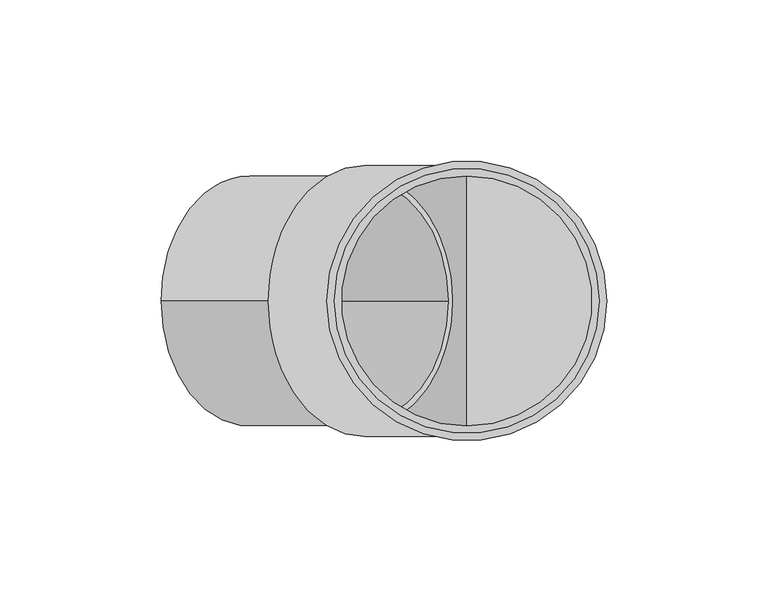
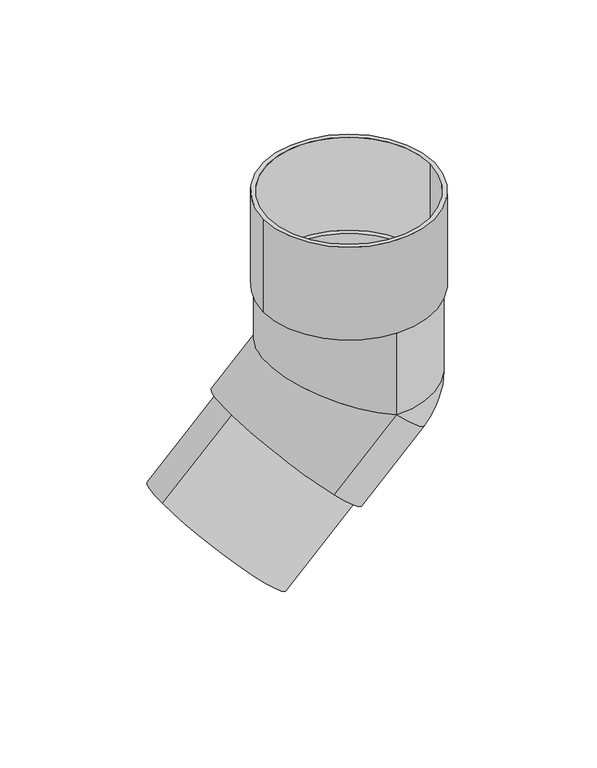
"""IFC4 building model written with IfcOpenShell, lengths in millimetres: proxy geometry, ⇲ Колено трубы 135 : ⇲ Колено трубы 135."""

import ifcopenshell
import ifcopenshell.guid

model = None  # the IFC model being written
_history = None  # IfcOwnerHistory: only IFC2X3 demands one
_inside = {}  # id of a spatial element -> (the spatial element, [elements in it])
_under = {}  # id of a project, library or spatial element -> (it, [spatial elements below it])
_declared = {}  # id of a project -> (the project, [libraries it declares])
_typed = {}  # id of a type object -> (the type object, [elements of that type])
_made_of = {}  # id of a material, layer set ... -> (it, [elements and type objects made of it])


def new_model(schema):
    """Start an empty IFC model of exactly this schema.

    Asked for "IFC4X3", IfcOpenShell would pick the latest addendum, in which some entities
    have other attributes; the version numbers below select the first issue.
    IFC2X3 requires an IfcOwnerHistory on every rooted entity: one is made here for all.
    """
    global model, _history
    if schema == "IFC4X3":
        model = ifcopenshell.file(schema_version=(4, 3, 0, 0))
    else:
        model = ifcopenshell.file(schema=schema)
    _inside.clear()
    _under.clear()
    _declared.clear()
    _typed.clear()
    _made_of.clear()
    _history = None
    if model.schema == "IFC2X3":
        org = make("IfcOrganization", Name="unknown")
        user = make(
            "IfcPersonAndOrganization",
            ThePerson=make("IfcPerson", FamilyName="unknown"),
            TheOrganization=org,
        )
        app = make(
            "IfcApplication",
            ApplicationDeveloper=org,
            Version="unknown",
            ApplicationFullName="unknown",
            ApplicationIdentifier="unknown",
        )
        _history = make(
            "IfcOwnerHistory",
            OwningUser=user,
            OwningApplication=app,
            ChangeAction="ADDED",
            CreationDate=0,
        )
    return model


def make(cls, **values):
    """One entity of the class cls with the attributes given. An attribute that is None is left unset."""
    return model.create_entity(
        cls, **{name: value for name, value in values.items() if value is not None}
    )


def rooted(cls, **values):
    """An entity with a GlobalId (a new one), such as an element, a storey or a relation."""
    return make(cls, GlobalId=ifcopenshell.guid.new(), OwnerHistory=_history, **values)


def si_unit(unit_type, name, prefix=None):
    """IfcSIUnit, for example si_unit("LENGTHUNIT", "METRE", prefix="MILLI")."""
    return make("IfcSIUnit", UnitType=unit_type, Prefix=prefix, Name=name)


def assignment(units):
    """IfcUnitAssignment: the units of a project."""
    return None if units is None else make("IfcUnitAssignment", Units=units)


def point(xyz):
    """IfcCartesianPoint."""
    return None if xyz is None else make("IfcCartesianPoint", Coordinates=xyz)


def direction(xyz):
    """IfcDirection."""
    return None if xyz is None else make("IfcDirection", DirectionRatios=xyz)


def frame(location, z_axis=None, x_axis=None):
    """IfcAxis2Placement3D, a coordinate frame: its origin and axes. An axis left out is left unset."""
    return make(
        "IfcAxis2Placement3D",
        Location=point(location),
        Axis=direction(z_axis),
        RefDirection=direction(x_axis),
    )


def origin():
    """The frame at (0, 0, 0) with its axes left unset."""
    return frame((0.0, 0.0, 0.0))


def origin_with_axes():
    """The frame at (0, 0, 0) with the z axis (0, 0, 1) and the x axis (1, 0, 0) written out."""
    return frame((0.0, 0.0, 0.0), z_axis=(0.0, 0.0, 1.0), x_axis=(1.0, 0.0, 0.0))


def place(relative_to, where):
    """IfcLocalPlacement: puts the frame where relative to a parent placement (None: the world)."""
    return make(
        "IfcLocalPlacement", PlacementRelTo=relative_to, RelativePlacement=where
    )


def context(
    kind, dimensions, precision=None, world=None, true_north=None, identifier=None
):
    """IfcGeometricRepresentationContext, for example the 3D "Model" context."""
    return make(
        "IfcGeometricRepresentationContext",
        ContextIdentifier=identifier,
        ContextType=kind,
        CoordinateSpaceDimension=dimensions,
        Precision=precision,
        WorldCoordinateSystem=world,
        TrueNorth=true_north,
    )


def project(units=None, contexts=None):
    """IfcProject with its units and contexts."""
    return rooted(
        "IfcProject",
        Name="project",
        RepresentationContexts=contexts,
        UnitsInContext=assignment(units),
    )


def spatial(cls, under=None, at=None, **own):
    """A site, building, storey or space (cls), placed at a placement, below another one or the project."""
    s = rooted(cls, ObjectPlacement=at, **own)
    if under is not None:
        _under.setdefault(under.id(), (under, []))[1].append(s)
    return s


def polyline(points):
    """IfcPolyline through the points."""
    return make("IfcPolyline", Points=[point(p) for p in points])


def circle_curve(where, radius):
    """IfcCircle in the frame where."""
    return make("IfcCircle", Position=where, Radius=radius)


def ellipse_curve(where, semi_axis1, semi_axis2):
    """IfcEllipse in the frame where."""
    return make(
        "IfcEllipse", Position=where, SemiAxis1=semi_axis1, SemiAxis2=semi_axis2
    )


def trimmed(basis, trim1, trim2, sense, master):
    """IfcTrimmedCurve: the piece of a basis curve between two trims."""
    return make(
        "IfcTrimmedCurve",
        BasisCurve=basis,
        Trim1=trim1,
        Trim2=trim2,
        SenseAgreement=sense,
        MasterRepresentation=master,
    )


def shape(context_of_items, identifier, shape_type, items):
    """IfcShapeRepresentation: the items that make up one representation, for example the "Body"."""
    return make(
        "IfcShapeRepresentation",
        ContextOfItems=context_of_items,
        RepresentationIdentifier=identifier,
        RepresentationType=shape_type,
        Items=items,
    )


def source(mapping_origin, context_of_items, identifier, shape_type, items):
    """IfcRepresentationMap: a shape defined once, which mapped items show again and again."""
    return make(
        "IfcRepresentationMap",
        MappingOrigin=mapping_origin,
        MappedRepresentation=shape(context_of_items, identifier, shape_type, items),
    )


def transform(
    local_origin,
    x_axis=None,
    y_axis=None,
    z_axis=None,
    scale=None,
    scale2=None,
    scale3=None,
    uniform=True,
):
    """IfcCartesianTransformationOperator3D, or its non-uniform kind. x_axis, y_axis, z_axis: its Axis1, 2, 3."""
    if uniform:
        return make(
            "IfcCartesianTransformationOperator3D",
            Axis1=direction(x_axis),
            Axis2=direction(y_axis),
            LocalOrigin=point(local_origin),
            Scale=scale,
            Axis3=direction(z_axis),
        )
    return make(
        "IfcCartesianTransformationOperator3DnonUniform",
        Axis1=direction(x_axis),
        Axis2=direction(y_axis),
        LocalOrigin=point(local_origin),
        Scale=scale,
        Axis3=direction(z_axis),
        Scale2=scale2,
        Scale3=scale3,
    )


def mapped(mapping_source, mapping_target):
    """IfcMappedItem: shows the shape of a source again, moved by a transform."""
    return make(
        "IfcMappedItem", MappingSource=mapping_source, MappingTarget=mapping_target
    )


def made_of(thing, what):
    """Note that an element or type object is made of a material, layer set ...; save() writes the relation."""
    if what is not None:
        _made_of.setdefault(what.id(), (what, []))[1].append(thing)
    return thing


def element(
    cls,
    number,
    at=None,
    inside=None,
    cuts=None,
    type_object=None,
    material=None,
    context=None,
    identifier="Body",
    shape_type=None,
    held_by="IfcProductDefinitionShape",
    body=None,
    shapes=None,
    **own,
):
    """One element of the class cls, such as IfcWall. Its Tag is "e" and its number.

    at: its placement. inside: the storey or other place that contains it. cuts: it is an
    opening in that element (IfcRelVoidsElement). A single representation is given by context,
    identifier, shape_type and body (its items); several are given by shapes. held_by: the class
    of the entity that holds the representations. save() writes the other relations.
    """
    e = rooted(cls, Tag="e%d" % number, ObjectPlacement=at, **own)
    if body is not None:
        shapes = [shape(context, identifier, shape_type, body)]
    if shapes is not None:
        e.Representation = make(held_by, Representations=shapes)
    if inside is not None:
        _inside.setdefault(inside.id(), (inside, []))[1].append(e)
    if cuts is not None:
        rooted(
            "IfcRelVoidsElement", RelatingBuildingElement=cuts, RelatedOpeningElement=e
        )
    if type_object is not None:
        _typed.setdefault(type_object.id(), (type_object, []))[1].append(e)
    return made_of(e, material)


def aggregate(whole, parts):
    """IfcRelAggregates: a whole, such as a stair, and the parts it consists of."""
    return rooted("IfcRelAggregates", RelatingObject=whole, RelatedObjects=parts)


def save(model, path):
    """Write the relations noted so far, then the file.

    IfcRelAggregates (storeys below a building ...), IfcRelContainedInSpatialStructure (elements
    in a storey), IfcRelDefinesByType, IfcRelAssociatesMaterial and IfcRelDeclares: one each for
    every whole, place, type object, material and project.
    """
    for whole, parts in _under.values():
        aggregate(whole, parts)
    for where, things in _inside.values():
        rooted(
            "IfcRelContainedInSpatialStructure",
            RelatedElements=things,
            RelatingStructure=where,
        )
    for kind, things in _typed.values():
        rooted("IfcRelDefinesByType", RelatedObjects=things, RelatingType=kind)
    for what, things in _made_of.values():
        rooted("IfcRelAssociatesMaterial", RelatedObjects=things, RelatingMaterial=what)
    for by, libraries in _declared.values():
        rooted("IfcRelDeclares", RelatingContext=by, RelatedDefinitions=libraries)
    model.write(path)


def plane_surface(at):
    """IfcPlane: the flat surface through the origin of the frame at, square to its z axis."""
    return make("IfcPlane", Position=at)


def cylinder_surface(at, radius):
    """IfcCylindricalSurface: all points at the distance radius from the z axis of the frame at."""
    return make("IfcCylindricalSurface", Position=at, Radius=radius)


def revolved_surface(curve, axis_point, axis_direction):
    """IfcSurfaceOfRevolution: the curve turned about the line through axis_point along axis_direction."""
    return make(
        "IfcSurfaceOfRevolution",
        SweptCurve=make("IfcArbitraryOpenProfileDef", ProfileType="CURVE", Curve=curve),
        AxisPosition=make("IfcAxis1Placement", Location=point(axis_point), Axis=direction(axis_direction)),
    )


def advanced_brep(points, edges, surfaces, faces):
    """IfcAdvancedBrep: a solid bounded by faces that lie on surfaces and meet in shared edges.

    An edge is (start, end): straight between two places in points (the first is 0);
    or (start, end, curve); or (start, end, curve, False) where it runs against its curve.
    A face is (place in surfaces, loops), or (place, loops, False) where it looks against
    its surface's normal. A loop lists edges by number (the first is 1), with a minus sign
    where the edge is run from its end to its start. The first loop is the outer one.
    """
    corners = [point(p) for p in points]
    vertices = [make("IfcVertexPoint", VertexGeometry=c) for c in corners]
    made = []
    for start, end, *more in edges:
        made.append(
            make(
                "IfcEdgeCurve",
                EdgeStart=vertices[start],
                EdgeEnd=vertices[end],
                EdgeGeometry=more[0] if more else make("IfcPolyline", Points=[corners[start], corners[end]]),
                SameSense=more[1] if len(more) > 1 else True,
            )
        )
    hull = []
    for where, loops, *sense in faces:
        bounds = []
        for j, loop in enumerate(loops):
            ring = [make("IfcOrientedEdge", EdgeElement=made[abs(k) - 1], Orientation=k > 0) for k in loop]
            bounds.append(
                make(
                    "IfcFaceOuterBound" if j == 0 else "IfcFaceBound",
                    Bound=make("IfcEdgeLoop", EdgeList=ring),
                    Orientation=True,
                )
            )
        hull.append(make("IfcAdvancedFace", Bounds=bounds, FaceSurface=surfaces[where], SameSense=sense[0] if sense else True))
    return make("IfcAdvancedBrep", Outer=make("IfcClosedShell", CfsFaces=hull))


def generic_models_0f0aad00(model_context):
    return source(origin(), model_context, "Body", "AdvancedBrep", [
        advanced_brep(
        [(41.1, 0.0, -50.0), (-41.1, 0.0, -50.0), (0.0, 38.8, -50.0), (0.0, -38.8, -50.0), (0.0, 42.0, -50.0), (0.0, 42.0, -95.0), (0.0, -42.0, -95.0), (0.0, -42.0, -50.0), (42.0, 0.0, -95.0), (0.0, 38.8, -95.0), (0.0, -38.8, -95.0), (-31.8198052, 42.0, -126.8198052), (-31.8198052, -42.0, -126.8198052), (-59.2555483, 0.0, -99.384062), (-31.8198052, -38.8, -126.8198052), (-4.384062, 0.0, -154.2555483), (-31.8198052, 38.8, -126.8198052), (29.6984848, 0.0, -124.6984848), (-31.8198052, 38.8, -126.8198052), (-4.384062, 0.0, -154.2555483), (-31.8198052, -38.8, -126.8198052), (-59.2555483, 0.0, -99.384062), (-43.4, 0.0, 0.0), (43.4, 0.0, 0.0), (-41.1, 0.0, 0.0), (41.1, 0.0, 0.0), (-43.4, 0.0, -50.0), (43.4, 0.0, -50.0), (-57.8413347, 0.0, -100.7982756), (-5.7982756, 0.0, -152.8413347), (-94.787868, 0.0, -134.9163817), (-39.9163817, 0.0, -189.787868), (-93.3736544, 0.0, -136.3305953), (-41.3305953, 0.0, -188.3736544)],
        [
            (0, 1, circle_curve(frame((0.0, 0.0, -50.0), z_axis=(0.0, 0.0, 1.0), x_axis=(1.0, 0.0, 0.0)), 41.1)),
            (1, 0, circle_curve(frame((0.0, 0.0, -50.0), z_axis=(0.0, 0.0, 1.0), x_axis=(1.0, 0.0, 0.0)), 41.1)),
            (2, 3, circle_curve(frame((0.0, 0.0, -50.0), z_axis=(0.0, 0.0, -1.0), x_axis=(0.0, -1.0, 0.0)), 38.8)),
            (3, 2, circle_curve(frame((0.0, 0.0, -50.0), z_axis=(0.0, 0.0, -1.0), x_axis=(0.0, -1.0, 0.0)), 38.8)),
            (4, 5),
            (5, 6, ellipse_curve(frame((0.0, 0.0, -95.0), z_axis=(0.38268343236509084, 0.0, 0.9238795325112863), x_axis=(-0.9238795325112863, 0.0, 0.38268343236509084)), 45.4604724, 42.0)),
            (6, 7),
            (7, 4, circle_curve(frame((0.0, 0.0, -50.0), z_axis=(0.0, 0.0, -1.0), x_axis=(0.0, -1.0, 0.0)), 42.0)),
            (4, 7, circle_curve(frame((0.0, 0.0, -50.0), z_axis=(0.0, 0.0, -1.0), x_axis=(0.0, -1.0, 0.0)), 42.0)),
            (6, 8, circle_curve(frame((0.0, 0.0, -95.0), z_axis=(0.0, 0.0, 1.0), x_axis=(0.0, -1.0, 0.0)), 42.0)),
            (8, 5, circle_curve(frame((0.0, 0.0, -95.0), z_axis=(0.0, 0.0, 1.0), x_axis=(0.0, -1.0, 0.0)), 42.0)),
            (2, 9),
            (9, 10, circle_curve(frame((0.0, 0.0, -95.0), z_axis=(0.0, 0.0, -1.0), x_axis=(0.0, -1.0, 0.0)), 38.8)),
            (10, 3),
            (10, 9, ellipse_curve(frame((0.0, 0.0, -95.0), z_axis=(-0.38268343236509084, 0.0, -0.9238795325112863), x_axis=(0.9238795325112863, 0.0, -0.38268343236509084)), 41.9968174, 38.8)),
            (11, 12, circle_curve(frame((-31.8198052, 0.0, -126.8198052), z_axis=(-0.7071067811865479, 0.0, -0.7071067811865471), x_axis=(0.0, -1.0, 0.0)), 42.0)),
            (12, 11, circle_curve(frame((-31.8198052, 0.0, -126.8198052), z_axis=(-0.7071067811865479, 0.0, -0.7071067811865471), x_axis=(0.0, -1.0, 0.0)), 42.0)),
            (13, 14, circle_curve(frame((-31.8198052, 0.0, -126.8198052), z_axis=(0.7071067811865457, 0.0, 0.7071067811865495), x_axis=(0.7071067811865495, 0.0, -0.7071067811865457)), 38.8)),
            (14, 15, circle_curve(frame((-31.8198052, 0.0, -126.8198052), z_axis=(0.7071067811865457, 0.0, 0.7071067811865495), x_axis=(0.7071067811865495, 0.0, -0.7071067811865457)), 38.8)),
            (15, 16, circle_curve(frame((-31.8198052, 0.0, -126.8198052), z_axis=(0.7071067811865457, 0.0, 0.7071067811865495), x_axis=(0.7071067811865495, 0.0, -0.7071067811865457)), 38.8)),
            (16, 13, circle_curve(frame((-31.8198052, 0.0, -126.8198052), z_axis=(0.7071067811865457, 0.0, 0.7071067811865495), x_axis=(0.7071067811865495, 0.0, -0.7071067811865457)), 38.8)),
            (5, 11),
            (12, 6),
            (5, 17, circle_curve(frame((0.0, 0.0, -95.0), z_axis=(-0.7071067811865479, 0.0, -0.7071067811865471), x_axis=(0.0, -1.0, 0.0)), 42.0)),
            (17, 6, circle_curve(frame((0.0, 0.0, -95.0), z_axis=(-0.7071067811865479, 0.0, -0.7071067811865471), x_axis=(0.0, -1.0, 0.0)), 42.0)),
            (9, 18),
            (18, 19, circle_curve(frame((-31.8198052, 0.0, -126.8198052), z_axis=(-0.7071067811865479, 0.0, -0.7071067811865471), x_axis=(0.0, -1.0, 0.0)), 38.8)),
            (19, 20, circle_curve(frame((-31.8198052, 0.0, -126.8198052), z_axis=(-0.7071067811865479, 0.0, -0.7071067811865471), x_axis=(0.0, -1.0, 0.0)), 38.8)),
            (20, 10),
            (10, 9, circle_curve(frame((0.0, 0.0, -95.0), z_axis=(0.7071067811865479, 0.0, 0.7071067811865471), x_axis=(0.0, -1.0, 0.0)), 38.8)),
            (20, 21, circle_curve(frame((-31.8198052, 0.0, -126.8198052), z_axis=(-0.7071067811865479, 0.0, -0.7071067811865471), x_axis=(0.0, -1.0, 0.0)), 38.8)),
            (21, 18, circle_curve(frame((-31.8198052, 0.0, -126.8198052), z_axis=(-0.7071067811865479, 0.0, -0.7071067811865471), x_axis=(0.0, -1.0, 0.0)), 38.8)),
            (9, 10),
            (17, 8, circle_curve(frame((0.0, 0.0, -95.0), z_axis=(0.0, -1.0, 0.0), x_axis=(1.0, 0.0, 0.0)), 42.0)),
            (22, 23, circle_curve(origin_with_axes(), 43.4)),
            (23, 22, circle_curve(origin_with_axes(), 43.4)),
            (24, 25, circle_curve(frame((0.0, 0.0, 0.0), z_axis=(0.0, 0.0, -1.0), x_axis=(1.0, 0.0, 0.0)), 41.1)),
            (25, 24, circle_curve(frame((0.0, 0.0, 0.0), z_axis=(0.0, 0.0, -1.0), x_axis=(1.0, 0.0, 0.0)), 41.1)),
            (26, 27, circle_curve(frame((0.0, 0.0, -50.0), z_axis=(0.0, 0.0, -1.0), x_axis=(1.0, 0.0, 0.0)), 43.4)),
            (27, 26, circle_curve(frame((0.0, 0.0, -50.0), z_axis=(0.0, 0.0, -1.0), x_axis=(1.0, 0.0, 0.0)), 43.4)),
            (24, 1),
            (0, 25),
            (22, 26),
            (27, 23),
            (28, 29, circle_curve(frame((-31.8198052, 0.0, -126.8198052), z_axis=(-0.7071067811865457, 0.0, -0.7071067811865495), x_axis=(0.7071067811865495, 0.0, -0.7071067811865457)), 36.8)),
            (29, 28, circle_curve(frame((-31.8198052, 0.0, -126.8198052), z_axis=(-0.7071067811865457, 0.0, -0.7071067811865495), x_axis=(0.7071067811865495, 0.0, -0.7071067811865457)), 36.8)),
            (30, 31, circle_curve(frame((-67.3521249, 0.0, -162.3521249), z_axis=(-0.7071067811865457, 0.0, -0.7071067811865495), x_axis=(0.7071067811865495, 0.0, -0.7071067811865457)), 38.8)),
            (31, 30, circle_curve(frame((-67.3521249, 0.0, -162.3521249), z_axis=(-0.7071067811865457, 0.0, -0.7071067811865495), x_axis=(0.7071067811865495, 0.0, -0.7071067811865457)), 38.8)),
            (32, 33, circle_curve(frame((-67.3521249, 0.0, -162.3521249), z_axis=(0.7071067811865457, 0.0, 0.7071067811865495), x_axis=(0.7071067811865495, 0.0, -0.7071067811865457)), 36.8)),
            (33, 32, circle_curve(frame((-67.3521249, 0.0, -162.3521249), z_axis=(0.7071067811865457, 0.0, 0.7071067811865495), x_axis=(0.7071067811865495, 0.0, -0.7071067811865457)), 36.8)),
            (31, 15),
            (13, 30),
            (28, 32),
            (33, 29),
        ],
        [
            plane_surface(frame((0.0, 0.0, -50.0), z_axis=(0.0, 0.0, 1.0), x_axis=(0.0, -1.0, 0.0))),
            cylinder_surface(frame((0.0, 0.0, -50.0), z_axis=(0.0, 0.0, 1.0), x_axis=(0.0, -1.0, 0.0)), 42.0),
            revolved_surface(polyline([(0.0, -38.8, -95.0), (0.0, -38.8, -50.0)]), (0.0, 0.0, -50.0), (0.0, 0.0, -1.0)),
            revolved_surface(polyline([(0.0, -38.8, -111.07148623104197), (0.0, -38.8, -50.0)]), (0.0, 0.0, -50.0), (0.0, 0.0, -1.0)),
            plane_surface(frame((-31.8198052, 0.0, -126.8198052), z_axis=(-0.7071067811865479, 0.0, -0.7071067811865471), x_axis=(0.0, -1.0, 0.0))),
            cylinder_surface(frame((0.0, 0.0, -95.0), z_axis=(0.7071067811865479, 0.0, 0.7071067811865471), x_axis=(0.0, -1.0, 0.0)), 42.0),
            revolved_surface(polyline([(-31.81980520000002, -38.8, -126.81980519999999), (0.0, -38.8, -95.0)]), (0.0, 0.0, -95.0), (-0.7071067811865479, 0.0, -0.7071067811865471)),
            revolved_surface(polyline([(-31.81980520000002, -38.8, -126.81980519999999), (11.364256897715961, -38.8, -83.63574310228405)]), (0.0, 0.0, -95.0), (-0.7071067811865479, 0.0, -0.7071067811865471)),
            plane_surface(frame((0.0, 2000.0, -95.0), z_axis=(0.0, 0.0, 1.0), x_axis=(1.0, 0.0, 0.0))),
            plane_surface(frame((0.0, 2000.0, -95.0), z_axis=(-0.707106781186547, 0.0, -0.7071067811865482), x_axis=(0.7071067811865482, 0.0, -0.707106781186547))),
            revolved_surface(trimmed(ellipse_curve(frame((0.0, 0.0, -95.0), z_axis=(0.0, 0.0, 1.0), x_axis=(1.0, 0.0, 0.0)), 42.0, 42.0), [point((0.0, -42.0, -95.0))], [point((42.0, 0.0, -95.0))], True, "CARTESIAN"), (0.0, 2000.0, -95.0), (0.0, 1.0, 0.0)),
            revolved_surface(trimmed(ellipse_curve(frame((0.0, 0.0, -95.0), z_axis=(0.0, 0.0, 1.0), x_axis=(1.0, 0.0, 0.0)), 42.0, 42.0), [point((42.0, 0.0, -95.0))], [point((0.0, 42.0, -95.0))], True, "CARTESIAN"), (0.0, 2000.0, -95.0), (0.0, 1.0, 0.0)),
            plane_surface(frame((41.1, 0.0, 0.0), z_axis=(0.0, 0.0, 1.0), x_axis=(0.0, -1.0, 0.0))),
            plane_surface(frame((41.1, 0.0, -50.0), z_axis=(0.0, 0.0, -1.0), x_axis=(0.0, 1.0, 0.0))),
            revolved_surface(polyline([(41.1, 0.0, -50.0), (41.1, 0.0, 0.0)]), (0.0, 0.0, -50.0), (0.0, 0.0, -1.0)),
            cylinder_surface(origin_with_axes(), 43.4),
            plane_surface(frame((-31.8198052, 0.0, -126.8198052), z_axis=(0.7071067811865457, 0.0, 0.7071067811865495), x_axis=(0.0, -1.0, 0.0))),
            plane_surface(frame((-67.3521249, 0.0, -162.3521249), z_axis=(-0.7071067811865457, 0.0, -0.7071067811865495), x_axis=(0.0, -1.0, 0.0))),
            cylinder_surface(frame((-31.8198052, 0.0, -126.8198052), z_axis=(0.7071067811865457, 0.0, 0.7071067811865495), x_axis=(0.7071067811865495, 0.0, -0.7071067811865457)), 38.8),
            revolved_surface(polyline([(-41.330595352334896, 0.0, -188.373654447665), (-5.7982756023349085, 0.0, -152.84133469766482)]), (-31.8198052, 0.0, -126.8198052), (-0.7071067811865457, 0.0, -0.7071067811865495)),
        ],
        [
            (0, [[1, 2], [3, 4]]),
            (1, [[5, 6, 7, 8]]),
            (1, [[-5, 9, -7, 10, 11]]),
            (2, [[-3, 12, 13, 14]]),
            (3, [[-4, -14, 15, -12]]),
            (4, [[16, 17], [18, 19, 20, 21]]),
            (5, [[-6, 22, -17, 23]]),
            (5, [[-16, -22, 24, 25, -23]]),
            (6, [[26, 27, 28, 29, 30]]),
            (7, [[-15, -29, 31, 32, -26]]),
            (8, [[33, -13]]),
            (9, [[-33, -30]]),
            (10, [[34, -10, -25]]),
            (11, [[-34, -24, -11]]),
            (12, [[35, 36], [37, 38]]),
            (13, [[39, 40], [-8, -9]]),
            (14, [[-37, 41, -1, 42]]),
            (14, [[-38, -42, -2, -41]]),
            (15, [[-35, 43, -40, 44]]),
            (15, [[-36, -44, -39, -43]]),
            (16, [[-27, -32, -31, -28], [45, 46]]),
            (17, [[47, 48], [49, 50]]),
            (18, [[-48, 51, -19, -18, 52]]),
            (18, [[-47, -52, -21, -20, -51]]),
            (19, [[-45, 53, -50, 54]]),
            (19, [[-46, -54, -49, -53]]),
        ],
    ),
    ])


if __name__ == "__main__":
    model = new_model("IFC4")
    model_context = context("Model", 3, world=origin())
    ifc_project = project(units=[si_unit("LENGTHUNIT", "METRE", prefix="MILLI")], contexts=[model_context])
    site = spatial("IfcSite", under=ifc_project)
    building = spatial("IfcBuilding", under=site)
    placement = place(None, origin())
    generic_models_shape = generic_models_0f0aad00(model_context)
    element("IfcBuildingElementProxy", 1, Name="⇲ Колено трубы 135 : ⇲ Колено трубы 135", ObjectType="⇲ Колено трубы 135 : ⇲ Колено трубы 135", at=placement, inside=building, context=model_context, shape_type="MappedRepresentation", body=[
        mapped(generic_models_shape, transform((0.0, 0.0, 0.0), x_axis=(1.0, 0.0, 0.0), y_axis=(0.0, 1.0, 0.0), z_axis=(0.0, 0.0, 1.0))),
    ])
    save(model, "model.ifc")

# Revit data of these elements
# Type "⇲ Колено трубы 135 : ⇲ Колено трубы 135"
#   Description = "Предназначено для изменения направления стока по трубе. Также применяется для обхода архитектурных элементов\r\nфасада"
#   Manufacturer = "ТехноНИКОЛЬ"
#   Model = "Комплектующие к водосточным системам"
#   URL = "https://tn-vodostok.ru/catalog/pvh/"
#   ADSK_Обозначение = "ТехноНИКОЛЬ"
#   ADSK_Наименование краткое = "Колено 135°"
#   ADSK_Наименование = "Колено трубы 135°"
#   ADSK_Масса_Текст = ""
#   ADSK_Марка = ""
#   ADSK_Код изделия = ""
#   ADSK_Завод-изготовитель = "ТехноНИКОЛЬ"
#   ADSK_Единица измерения = "шт."
#   ADSK_Группирование = "Комплектующие к водосточным системам"
#   ADSK_URL страницы изделия = "https://tn-vodostok.ru/catalog/pvh/"
#   ADSK_URL документации изделия = "https://tn-vodostok.ru/upload/iblock/c42/c427963cb77eb5c3c51f0cfb870e9e52.pdf"
#   Угол поворота хомута [instance default] = 0.00°
#   ADSK_Размер_Ширина = 143.3 mm
#   ADSK_Размер_Диаметр = 82.2 mm
#   ADSK_Размер_Высота = 190 mm
#   ADSK_Количество = 1
#   ADSK_Материал [instance default] = TN_Пластик_Коричневый_RAL8019
#   Default Elevation = 0
# Element 1 (IfcBuildingElementProxy, "⇲ Колено трубы 135 : ⇲ Колено трубы 135")
#   Materials on its faces: "TN_Пластик_Коричневый_RAL8019"
# Materials
#   "TN_Пластик_Коричневый_RAL8019": class "Типовые", colour RGB 61 54 53, transparency 0, Cost = 0
